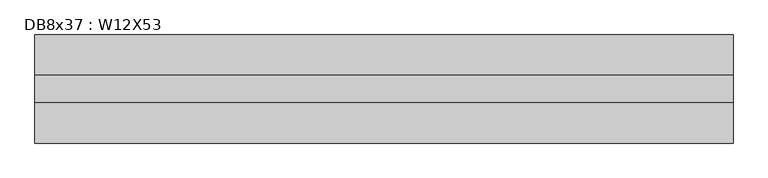
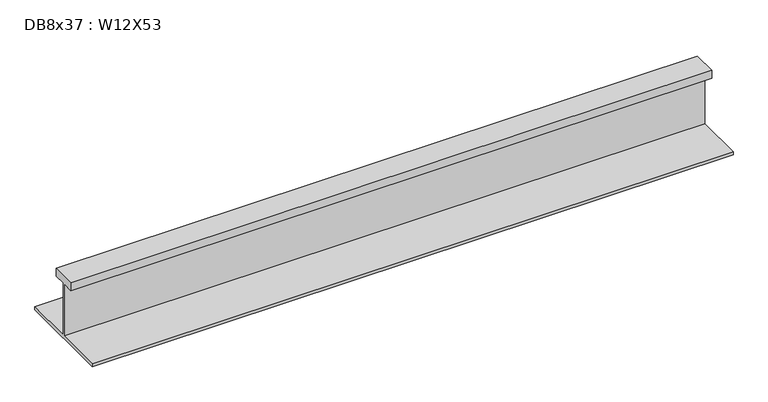
"""IFC4 building model written with IfcOpenShell, lengths in millimetres: beam geometry, DB8x37 : W12X53."""

from ifc_helpers import new_model, si_unit, frame, origin, place, context, project, spatial, polyline, outline, extrude, source, transform, mapped, element, save


def db8x37_w12x53_7850b3a4(model_context):
    return source(origin(), model_context, "Body", "SweptSolid", [
        extrude(outline(polyline([(38.1, 145.415), (38.1, 120.015), (2.921, 120.015), (2.921, -48.4505), (152.4, -48.4505), (152.4, -58.1025), (-152.4, -58.1025), (-152.4, -48.4505), (-2.921, -48.4505), (-2.921, 120.015), (-38.1, 120.015), (-38.1, 145.415), (38.1, 145.415)])), frame((-977.8999994, 0.0, 0.0), z_axis=(1.0, 0.0, 0.0), x_axis=(0.0, 1.0, 0.0)), (0.0, 0.0, 1.0), 1968.4999994),
    ])


if __name__ == "__main__":
    model = new_model("IFC4")
    model_context = context("Model", 3, world=origin())
    ifc_project = project(units=[si_unit("LENGTHUNIT", "METRE", prefix="MILLI")], contexts=[model_context])
    site = spatial("IfcSite", under=ifc_project)
    building = spatial("IfcBuilding", under=site)
    placement = place(None, origin())
    db8x37_w12x53_shape = db8x37_w12x53_7850b3a4(model_context)
    element("IfcBeam", 1, ObjectType="DB8x37 : W12X53", at=placement, inside=building, context=model_context, shape_type="MappedRepresentation", body=[
        mapped(db8x37_w12x53_shape, transform((0.0, 0.0, 0.0), x_axis=(1.0, 0.0, 0.0), y_axis=(0.0, 1.0, 0.0), z_axis=(0.0, 0.0, 1.0))),
    ])
    save(model, "model.ifc")

# Revit data of these elements
# Type "DB8x37 : W12X53"
#   Assembly Code = "B10"
#   W = 53
#   Length [instance default] = 5' - 0"
#   bf = 0' - 10"
#   d = 1' - 0.1"
#   k = 0' - 1 3/8"
#   k2 = 0' - 0.8"
#   tf = 0' - 0.575"
#   tw = 0' - 0.345"
#   A = 0.108333 SF
#   Structural Material [instance default] = Steel ASTM A992
# Element 1 (IfcBeam, "DB8x37 : W12X53")
#   Materials on its faces: "Steel ASTM A992"
# Materials
#   "Steel ASTM A992": class "Metal", colour RGB 199 199 199, transparency 0, Description = "Structural steel 50ksi", Cost = 0
